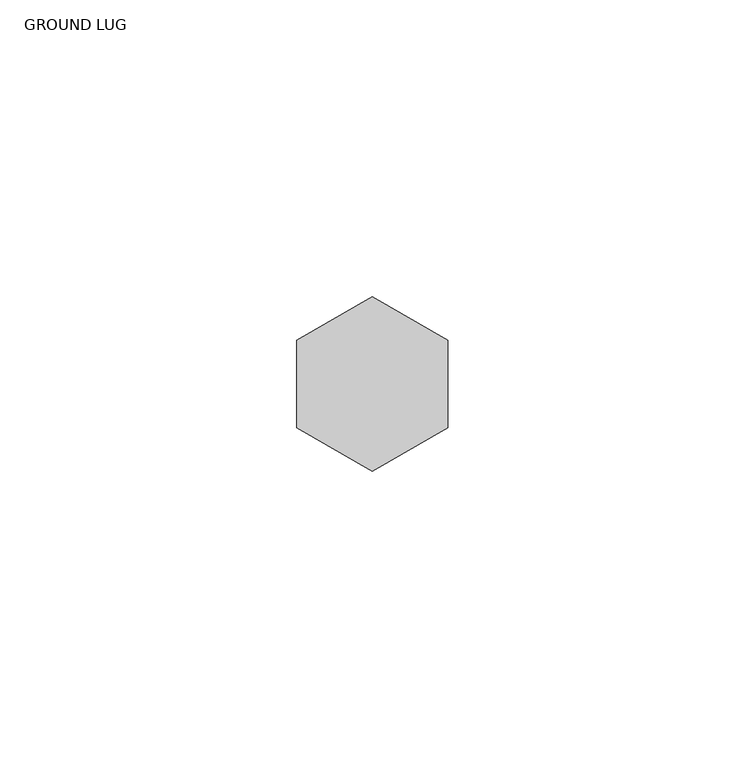
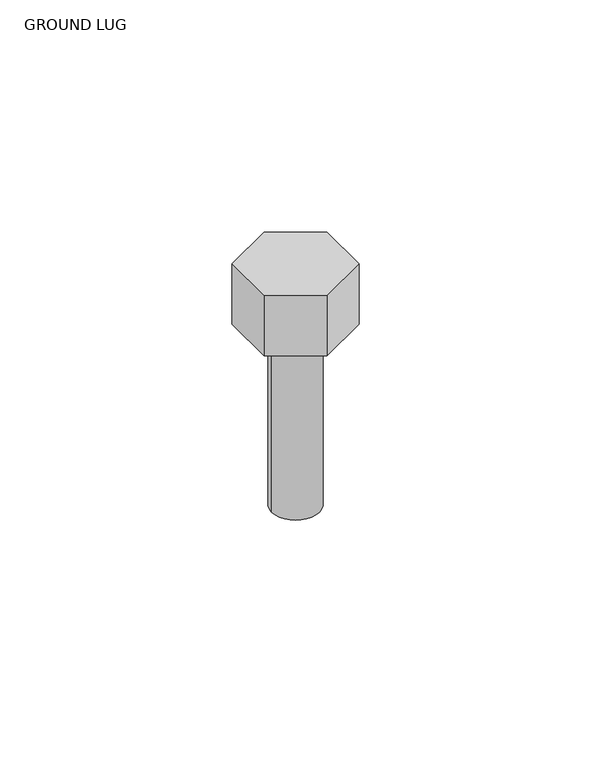
"""IFC4 building model written with IfcOpenShell, lengths in millimetres: proxy geometry, 050523 - W_P_C - Fastenings - Lag Bolt or Thru Bolt : GROUND LUG."""

from ifc_helpers import new_model, si_unit, point, frame, origin, origin_with_axes, origin_2d, place, context, project, spatial, polyline, circle_curve, trimmed, segment, composite_curve, outline, extrude, source, transform, mapped, element, save


def ground_lug_776e72c6(model_context):
    return source(origin(), model_context, "Body", "SweptSolid", [
        extrude(outline(polyline([(-12.7, 7.3323484), (0.0, 14.6646968), (12.7, 7.3323484), (12.7, -7.3323484), (0.0, -14.6646968), (-12.7, -7.3323484), (-12.7, 7.3323484)])), origin_with_axes(), (0.0, 0.0, 1.0), 17.065625),
        extrude(outline(composite_curve([segment(trimmed(circle_curve(origin_2d(), 6.35), [point((-6.35, 0.0))], [point((6.35, 0.0))], False, "CARTESIAN"), True, "CONTINUOUS"), segment(trimmed(circle_curve(origin_2d(), 6.35), [point((6.35, 0.0))], [point((-6.35, 0.0))], False, "CARTESIAN"), True, "CONTINUOUS")], self_intersect=False)), frame((0.0, 0.0, -50.8), z_axis=(0.0, 0.0, 1.0), x_axis=(1.0, 0.0, 0.0)), (0.0, 0.0, 1.0), 50.8),
    ])


if __name__ == "__main__":
    model = new_model("IFC4")
    model_context = context("Model", 3, world=origin())
    ifc_project = project(units=[si_unit("LENGTHUNIT", "METRE", prefix="MILLI")], contexts=[model_context])
    site = spatial("IfcSite", under=ifc_project)
    building = spatial("IfcBuilding", under=site)
    placement = place(None, origin())
    ground_lug_shape = ground_lug_776e72c6(model_context)
    element("IfcBuildingElementProxy", 1, Name="050523 - W_P_C - Fastenings - Lag Bolt or Thru Bolt : GROUND LUG", ObjectType="050523 - W_P_C - Fastenings - Lag Bolt or Thru Bolt : GROUND LUG", at=placement, inside=building, context=model_context, shape_type="MappedRepresentation", body=[
        mapped(ground_lug_shape, transform((0.0, 0.0, 0.0), x_axis=(1.0, 0.0, 0.0), y_axis=(0.0, 1.0, 0.0), z_axis=(0.0, 0.0, 1.0))),
    ])
    save(model, "model.ifc")

# Revit data of these elements
# Type "050523 - W_P_C - Fastenings - Lag Bolt or Thru Bolt : GROUND LUG"
#   Thickness_of_Substrate [instance default] = 0' - 1"
#   Side = 0' - 0 37/64"
#   Radius = 0' - 0 1/4"
#   Length = 0' - 2"
#   Head Size = 0' - 1"
#   Head Radius = 0' - 0 1/2"
#   Head Height = 0' - 0 43/64"
#   Diameter = 0' - 0 1/2"
#   Default Elevation = 4' - 0"
#   Nut_Visibility [instance default] = yes
#   Bolt Material (Size) = GROUND WIRE BOLTED TO POLE'S GROUND LUG
# Element 1 (IfcBuildingElementProxy, "050523 - W_P_C - Fastenings - Lag Bolt or Thru Bolt : GROUND LUG")
#   Thickness_of_Substrate = 3' - 0"
#   Nut_Visibility = no
#   Materials on its faces: "GROUND WIRE BOLTED TO POLE'S GROUND LUG"
# Materials
#   "GROUND WIRE BOLTED TO POLE'S GROUND LUG": class "Generic", colour RGB 120 120 120, transparency 0, Cost = 0
